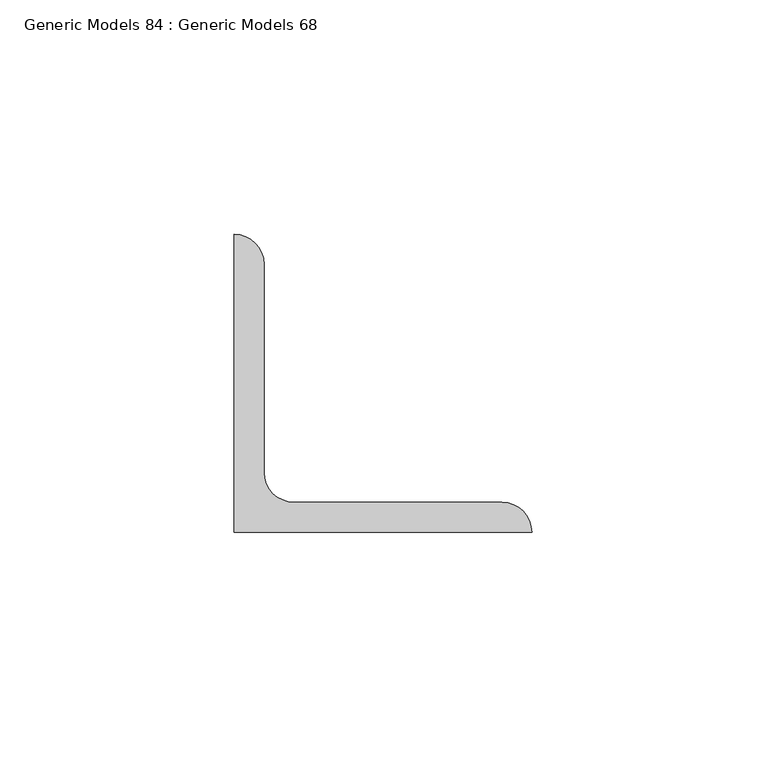
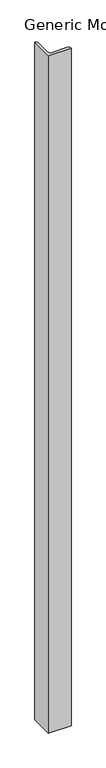
"""IFC4 building model written with IfcOpenShell, lengths in millimetres: proxy geometry, Generic Models 84 : Generic Models 68."""

from ifc_helpers import new_model, si_unit, point, frame, frame_2d, origin, place, context, project, spatial, polyline, circle_curve, trimmed, segment, composite_curve, outline, extrude, source, transform, mapped, element, save


def generic_models_84_generic_models_68_d4773e7f(model_context):
    return source(origin(), model_context, "Body", "SweptSolid", [
        extrude(outline(composite_curve([segment(polyline([(20530.4116945, 19715.2264581), (20530.4116945, 19778.7264581)]), True, "CONTINUOUS"), segment(trimmed(circle_curve(frame_2d((20530.4116945, 19772.3764581)), 6.35), [point((20530.4116945, 19778.7264581))], [point((20536.7616945, 19772.3764581))], False, "CARTESIAN"), True, "CONTINUOUS"), segment(polyline([(20536.7616945, 19772.3764581), (20536.7616945, 19727.9264581)]), True, "CONTINUOUS"), segment(trimmed(circle_curve(frame_2d((20543.1116945, 19727.9264581)), 6.35), [point((20536.7616945, 19727.9264581))], [point((20543.1116945, 19721.5764581))], True, "CARTESIAN"), True, "CONTINUOUS"), segment(polyline([(20543.1116945, 19721.5764581), (20587.5616945, 19721.5764581)]), True, "CONTINUOUS"), segment(trimmed(circle_curve(frame_2d((20587.5616945, 19715.2264581)), 6.35), [point((20587.5616945, 19721.5764581))], [point((20593.9116945, 19715.2264581))], False, "CARTESIAN"), True, "CONTINUOUS"), segment(polyline([(20593.9116945, 19715.2264581), (20530.4116945, 19715.2264581)]), True, "CONTINUOUS")], self_intersect=False)), frame((0.0, 0.0, 265402.3336948), z_axis=(0.0, 0.0, 1.0), x_axis=(1.0, 0.0, 0.0)), (0.0, 0.0, 1.0), 1984.375),
    ])


if __name__ == "__main__":
    model = new_model("IFC4")
    model_context = context("Model", 3, world=origin())
    ifc_project = project(units=[si_unit("LENGTHUNIT", "METRE", prefix="MILLI")], contexts=[model_context])
    site = spatial("IfcSite", under=ifc_project)
    building = spatial("IfcBuilding", under=site)
    placement = place(None, origin())
    generic_models_84_generic_models_68_shape = generic_models_84_generic_models_68_d4773e7f(model_context)
    element("IfcBuildingElementProxy", 1, Name="Generic Models 84 : Generic Models 68", ObjectType="Generic Models 84 : Generic Models 68", at=placement, inside=building, context=model_context, shape_type="MappedRepresentation", body=[
        mapped(generic_models_84_generic_models_68_shape, transform((0.0, 0.0, 0.0), x_axis=(1.0, 0.0, 0.0), y_axis=(0.0, 1.0, 0.0), z_axis=(0.0, 0.0, 1.0))),
    ])
    save(model, "model.ifc")

# Revit data of these elements
# Element 1 (IfcBuildingElementProxy, "Generic Models 84 : Generic Models 68")
#   Materials on its faces: "INTERMITTENT FENCE POST:  (2) BACK/BACK GALV. ANGLES (L2 1/2 X 2 1/2 X 1/4\") - NO FOOTING"
# Materials
#   "INTERMITTENT FENCE POST:  (2) BACK/BACK GALV. ANGLES (L2 1/2 X 2 1/2 X 1/4\") - NO FOOTING": class "Unassigned", colour RGB 211 211 211, transparency 0, Cost = 0
